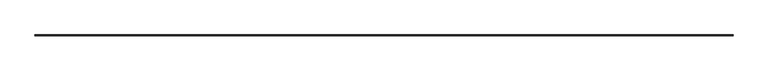
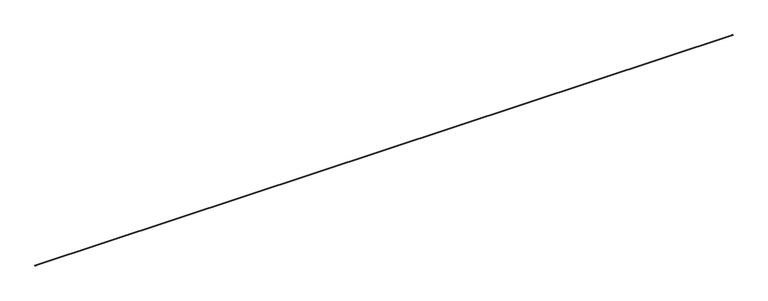
"""IFC4 building model written with IfcOpenShell, lengths in millimetres: proxy geometry, Generic Models 7:Generic Models 1:6:Generic Models 1:6 : Generic Models 7:Generic Models 1:337419:21 : Generic Models 7:Generic Models 1:6:Generic Models 1:6 : Generic Models 7:Generic Models 1:337419:312901."""

import ifcopenshell
import ifcopenshell.guid

model = None  # the IFC model being written
_history = None  # IfcOwnerHistory: only IFC2X3 demands one
_inside = {}  # id of a spatial element -> (the spatial element, [elements in it])
_under = {}  # id of a project, library or spatial element -> (it, [spatial elements below it])
_declared = {}  # id of a project -> (the project, [libraries it declares])
_typed = {}  # id of a type object -> (the type object, [elements of that type])
_made_of = {}  # id of a material, layer set ... -> (it, [elements and type objects made of it])


def new_model(schema):
    """Start an empty IFC model of exactly this schema.

    Asked for "IFC4X3", IfcOpenShell would pick the latest addendum, in which some entities
    have other attributes; the version numbers below select the first issue.
    IFC2X3 requires an IfcOwnerHistory on every rooted entity: one is made here for all.
    """
    global model, _history
    if schema == "IFC4X3":
        model = ifcopenshell.file(schema_version=(4, 3, 0, 0))
    else:
        model = ifcopenshell.file(schema=schema)
    _inside.clear()
    _under.clear()
    _declared.clear()
    _typed.clear()
    _made_of.clear()
    _history = None
    if model.schema == "IFC2X3":
        org = make("IfcOrganization", Name="unknown")
        user = make(
            "IfcPersonAndOrganization",
            ThePerson=make("IfcPerson", FamilyName="unknown"),
            TheOrganization=org,
        )
        app = make(
            "IfcApplication",
            ApplicationDeveloper=org,
            Version="unknown",
            ApplicationFullName="unknown",
            ApplicationIdentifier="unknown",
        )
        _history = make(
            "IfcOwnerHistory",
            OwningUser=user,
            OwningApplication=app,
            ChangeAction="ADDED",
            CreationDate=0,
        )
    return model


def make(cls, **values):
    """One entity of the class cls with the attributes given. An attribute that is None is left unset."""
    return model.create_entity(
        cls, **{name: value for name, value in values.items() if value is not None}
    )


def rooted(cls, **values):
    """An entity with a GlobalId (a new one), such as an element, a storey or a relation."""
    return make(cls, GlobalId=ifcopenshell.guid.new(), OwnerHistory=_history, **values)


def si_unit(unit_type, name, prefix=None):
    """IfcSIUnit, for example si_unit("LENGTHUNIT", "METRE", prefix="MILLI")."""
    return make("IfcSIUnit", UnitType=unit_type, Prefix=prefix, Name=name)


def assignment(units):
    """IfcUnitAssignment: the units of a project."""
    return None if units is None else make("IfcUnitAssignment", Units=units)


def point(xyz):
    """IfcCartesianPoint."""
    return None if xyz is None else make("IfcCartesianPoint", Coordinates=xyz)


def direction(xyz):
    """IfcDirection."""
    return None if xyz is None else make("IfcDirection", DirectionRatios=xyz)


def frame(location, z_axis=None, x_axis=None):
    """IfcAxis2Placement3D, a coordinate frame: its origin and axes. An axis left out is left unset."""
    return make(
        "IfcAxis2Placement3D",
        Location=point(location),
        Axis=direction(z_axis),
        RefDirection=direction(x_axis),
    )


def frame_2d(location, x_axis=None):
    """IfcAxis2Placement2D, a coordinate frame in the plane: its origin and x axis."""
    return make(
        "IfcAxis2Placement2D", Location=point(location), RefDirection=direction(x_axis)
    )


def origin():
    """The frame at (0, 0, 0) with its axes left unset."""
    return frame((0.0, 0.0, 0.0))


def place(relative_to, where):
    """IfcLocalPlacement: puts the frame where relative to a parent placement (None: the world)."""
    return make(
        "IfcLocalPlacement", PlacementRelTo=relative_to, RelativePlacement=where
    )


def context(
    kind, dimensions, precision=None, world=None, true_north=None, identifier=None
):
    """IfcGeometricRepresentationContext, for example the 3D "Model" context."""
    return make(
        "IfcGeometricRepresentationContext",
        ContextIdentifier=identifier,
        ContextType=kind,
        CoordinateSpaceDimension=dimensions,
        Precision=precision,
        WorldCoordinateSystem=world,
        TrueNorth=true_north,
    )


def project(units=None, contexts=None):
    """IfcProject with its units and contexts."""
    return rooted(
        "IfcProject",
        Name="project",
        RepresentationContexts=contexts,
        UnitsInContext=assignment(units),
    )


def spatial(cls, under=None, at=None, **own):
    """A site, building, storey or space (cls), placed at a placement, below another one or the project."""
    s = rooted(cls, ObjectPlacement=at, **own)
    if under is not None:
        _under.setdefault(under.id(), (under, []))[1].append(s)
    return s


def circle_curve(where, radius):
    """IfcCircle in the frame where."""
    return make("IfcCircle", Position=where, Radius=radius)


def trimmed(basis, trim1, trim2, sense, master):
    """IfcTrimmedCurve: the piece of a basis curve between two trims."""
    return make(
        "IfcTrimmedCurve",
        BasisCurve=basis,
        Trim1=trim1,
        Trim2=trim2,
        SenseAgreement=sense,
        MasterRepresentation=master,
    )


def segment(curve, same_sense, transition):
    """IfcCompositeCurveSegment."""
    return make(
        "IfcCompositeCurveSegment",
        Transition=transition,
        SameSense=same_sense,
        ParentCurve=curve,
    )


def composite_curve(segments, self_intersect=None):
    """IfcCompositeCurve: segments joined end to end."""
    return make("IfcCompositeCurve", Segments=segments, SelfIntersect=self_intersect)


def outline(outer, holes=None, kind="AREA"):
    """IfcArbitraryClosedProfileDef: a profile drawn as a closed curve; with holes, ...WithVoids."""
    if holes is None:
        return make("IfcArbitraryClosedProfileDef", ProfileType=kind, OuterCurve=outer)
    return make(
        "IfcArbitraryProfileDefWithVoids",
        ProfileType=kind,
        OuterCurve=outer,
        InnerCurves=holes,
    )


def extrude(swept, where, along, depth):
    """IfcExtrudedAreaSolid: the profile swept, set in the frame where, extruded along a direction by depth."""
    return make(
        "IfcExtrudedAreaSolid",
        SweptArea=swept,
        Position=where,
        ExtrudedDirection=direction(along),
        Depth=depth,
    )


def shape(context_of_items, identifier, shape_type, items):
    """IfcShapeRepresentation: the items that make up one representation, for example the "Body"."""
    return make(
        "IfcShapeRepresentation",
        ContextOfItems=context_of_items,
        RepresentationIdentifier=identifier,
        RepresentationType=shape_type,
        Items=items,
    )


def source(mapping_origin, context_of_items, identifier, shape_type, items):
    """IfcRepresentationMap: a shape defined once, which mapped items show again and again."""
    return make(
        "IfcRepresentationMap",
        MappingOrigin=mapping_origin,
        MappedRepresentation=shape(context_of_items, identifier, shape_type, items),
    )


def transform(
    local_origin,
    x_axis=None,
    y_axis=None,
    z_axis=None,
    scale=None,
    scale2=None,
    scale3=None,
    uniform=True,
):
    """IfcCartesianTransformationOperator3D, or its non-uniform kind. x_axis, y_axis, z_axis: its Axis1, 2, 3."""
    if uniform:
        return make(
            "IfcCartesianTransformationOperator3D",
            Axis1=direction(x_axis),
            Axis2=direction(y_axis),
            LocalOrigin=point(local_origin),
            Scale=scale,
            Axis3=direction(z_axis),
        )
    return make(
        "IfcCartesianTransformationOperator3DnonUniform",
        Axis1=direction(x_axis),
        Axis2=direction(y_axis),
        LocalOrigin=point(local_origin),
        Scale=scale,
        Axis3=direction(z_axis),
        Scale2=scale2,
        Scale3=scale3,
    )


def mapped(mapping_source, mapping_target):
    """IfcMappedItem: shows the shape of a source again, moved by a transform."""
    return make(
        "IfcMappedItem", MappingSource=mapping_source, MappingTarget=mapping_target
    )


def made_of(thing, what):
    """Note that an element or type object is made of a material, layer set ...; save() writes the relation."""
    if what is not None:
        _made_of.setdefault(what.id(), (what, []))[1].append(thing)
    return thing


def element(
    cls,
    number,
    at=None,
    inside=None,
    cuts=None,
    type_object=None,
    material=None,
    context=None,
    identifier="Body",
    shape_type=None,
    held_by="IfcProductDefinitionShape",
    body=None,
    shapes=None,
    **own,
):
    """One element of the class cls, such as IfcWall. Its Tag is "e" and its number.

    at: its placement. inside: the storey or other place that contains it. cuts: it is an
    opening in that element (IfcRelVoidsElement). A single representation is given by context,
    identifier, shape_type and body (its items); several are given by shapes. held_by: the class
    of the entity that holds the representations. save() writes the other relations.
    """
    e = rooted(cls, Tag="e%d" % number, ObjectPlacement=at, **own)
    if body is not None:
        shapes = [shape(context, identifier, shape_type, body)]
    if shapes is not None:
        e.Representation = make(held_by, Representations=shapes)
    if inside is not None:
        _inside.setdefault(inside.id(), (inside, []))[1].append(e)
    if cuts is not None:
        rooted(
            "IfcRelVoidsElement", RelatingBuildingElement=cuts, RelatedOpeningElement=e
        )
    if type_object is not None:
        _typed.setdefault(type_object.id(), (type_object, []))[1].append(e)
    return made_of(e, material)


def aggregate(whole, parts):
    """IfcRelAggregates: a whole, such as a stair, and the parts it consists of."""
    return rooted("IfcRelAggregates", RelatingObject=whole, RelatedObjects=parts)


def save(model, path):
    """Write the relations noted so far, then the file.

    IfcRelAggregates (storeys below a building ...), IfcRelContainedInSpatialStructure (elements
    in a storey), IfcRelDefinesByType, IfcRelAssociatesMaterial and IfcRelDeclares: one each for
    every whole, place, type object, material and project.
    """
    for whole, parts in _under.values():
        aggregate(whole, parts)
    for where, things in _inside.values():
        rooted(
            "IfcRelContainedInSpatialStructure",
            RelatedElements=things,
            RelatingStructure=where,
        )
    for kind, things in _typed.values():
        rooted("IfcRelDefinesByType", RelatedObjects=things, RelatingType=kind)
    for what, things in _made_of.values():
        rooted("IfcRelAssociatesMaterial", RelatedObjects=things, RelatingMaterial=what)
    for by, libraries in _declared.values():
        rooted("IfcRelDeclares", RelatingContext=by, RelatedDefinitions=libraries)
    model.write(path)


def generic_models_42f976ce(model_context):
    return source(origin(), model_context, "Body", "SweptSolid", [
        extrude(outline(composite_curve([segment(trimmed(circle_curve(frame_2d((-578733.9312882, -117.5511262)), 6.35), [point((-578727.5812882, -117.5511262))], [point((-578740.2812882, -117.5511262))], False, "CARTESIAN"), True, "CONTINUOUS"), segment(trimmed(circle_curve(frame_2d((-578733.9312882, -117.5511262)), 6.35), [point((-578740.2812882, -117.5511262))], [point((-578727.5812882, -117.5511262))], False, "CARTESIAN"), True, "CONTINUOUS")], self_intersect=False)), frame((557771.6867239, 0.0, 0.0), z_axis=(1.0, 0.0, 0.0), x_axis=(0.0, 1.0, 0.0)), (0.0, 0.0, 1.0), 109559.725),
        extrude(outline(composite_curve([segment(trimmed(circle_curve(frame_2d((-578632.3312882, -117.5511262)), 6.35), [point((-578625.9812882, -117.5511262))], [point((-578638.6812882, -117.5511262))], False, "CARTESIAN"), True, "CONTINUOUS"), segment(trimmed(circle_curve(frame_2d((-578632.3312882, -117.5511262)), 6.35), [point((-578638.6812882, -117.5511262))], [point((-578625.9812882, -117.5511262))], False, "CARTESIAN"), True, "CONTINUOUS")], self_intersect=False)), frame((557771.6867239, 0.0, 0.0), z_axis=(1.0, 0.0, 0.0), x_axis=(0.0, 1.0, 0.0)), (0.0, 0.0, 1.0), 109559.725),
    ])


if __name__ == "__main__":
    model = new_model("IFC4")
    model_context = context("Model", 3, world=origin())
    ifc_project = project(units=[si_unit("LENGTHUNIT", "METRE", prefix="MILLI")], contexts=[model_context])
    site = spatial("IfcSite", under=ifc_project)
    building = spatial("IfcBuilding", under=site)
    placement = place(None, origin())
    generic_models_shape = generic_models_42f976ce(model_context)
    element("IfcBuildingElementProxy", 1, Name="Generic Models 7:Generic Models 1:6:Generic Models 1:6 : Generic Models 7:Generic Models 1:337419:21 : Generic Models 7:Generic Models 1:6:Generic Models 1:6 : Generic Models 7:Generic Models 1:337419:312901", ObjectType="Generic Models 7:Generic Models 1:6:Generic Models 1:6 : Generic Models 7:Generic Models 1:337419:21 : Generic Models 7:Generic Models 1:6:Generic Models 1:6 : Generic Models 7:Generic Models 1:337419:312901", at=placement, inside=building, context=model_context, shape_type="MappedRepresentation", body=[
        mapped(generic_models_shape, transform((0.0, 0.0, 0.0), x_axis=(1.0, 0.0, 0.0), y_axis=(0.0, 1.0, 0.0), z_axis=(0.0, 0.0, 1.0))),
    ])
    save(model, "model.ifc")

# Revit data of these elements
# Type "Generic Models 7:Generic Models 1:6:Generic Models 1:6 : Generic Models 7:Generic Models 1:337419:21 : Generic Models 7:Generic Models 1:6:Generic Models 1:6 : Generic Models 7:Generic Models 1:337419:312901"
#   NameOverride = "Generic Models 7:Generic Models 1:6:Generic Models 1:6 : Generic Models 7:Generic Models 1:337419:312901"
#   ObjectTypeOverride = "Generic Models 1:6 : Generic Models 7:Generic Models 1:337419"
#   Reference = "Generic Models 1"
#   Tag = "312901"
# Element 1 (IfcBuildingElementProxy, "Generic Models 7:Generic Models 1:6:Generic Models 1:6 : Generic Models 7:Generic Models 1:337419:21 : Generic Models 7:Generic Models 1:6:Generic Models 1:6 : Generic Models 7:Generic Models 1:337419:312901")
#   Materials on its faces: "RADIANT TUBING"
# Materials
#   "RADIANT TUBING": class "Generic", colour RGB 215 211 94, transparency 0, Cost = 0
